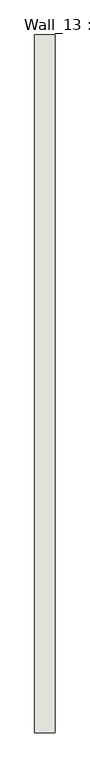
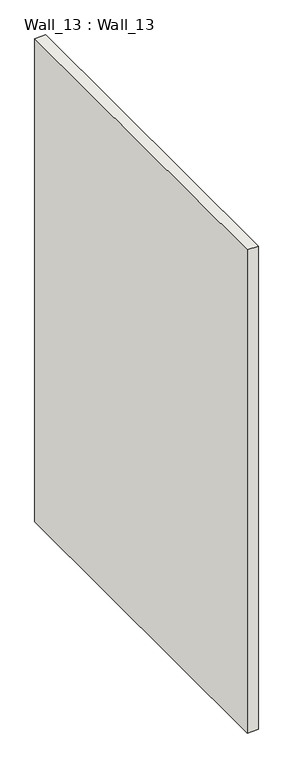
"""IFC4 building model written with IfcOpenShell, lengths in millimetres: wall geometry, Wall_13 : Wall_13."""

from ifc_helpers import new_model, si_unit, origin, origin_with_axes, place, context, project, spatial, polyline, outline, extrude, source, transform, mapped, element, save


def wall_13_wall_13_25ff5e73(model_context):
    return source(origin(), model_context, "Body", "SweptSolid", [
        extrude(outline(polyline([(5040.0, 3770.0), (5040.0, 380.0), (4940.0, 380.0), (4940.0, 3770.0), (5040.0, 3770.0)])), origin_with_axes(), (0.0, 0.0, 1.0), 4700.0),
    ])


if __name__ == "__main__":
    model = new_model("IFC4")
    model_context = context("Model", 3, world=origin())
    ifc_project = project(units=[si_unit("LENGTHUNIT", "METRE", prefix="MILLI")], contexts=[model_context])
    site = spatial("IfcSite", under=ifc_project)
    building = spatial("IfcBuilding", under=site)
    placement = place(None, origin())
    wall_13_wall_13_shape = wall_13_wall_13_25ff5e73(model_context)
    element("IfcWall", 1, ObjectType="Wall_13 : Wall_13", at=placement, inside=building, context=model_context, shape_type="MappedRepresentation", body=[
        mapped(wall_13_wall_13_shape, transform((0.0, 0.0, 0.0), x_axis=(1.0, 0.0, 0.0), y_axis=(0.0, 1.0, 0.0), z_axis=(0.0, 0.0, 1.0))),
    ])
    save(model, "model.ifc")

# Revit data of these elements
# Type "Wall_13 : Wall_13"
#   NameOverride = "Wall_13"
# Element 1 (IfcWall, "Wall_13 : Wall_13")
#   Materials on its faces: "IfcSurfaceStyle #33"
# Materials
#   "IfcSurfaceStyle #33": class "Unassigned", colour RGB 214 214 214, transparency 0
